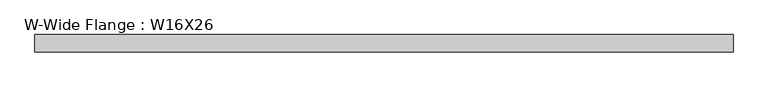
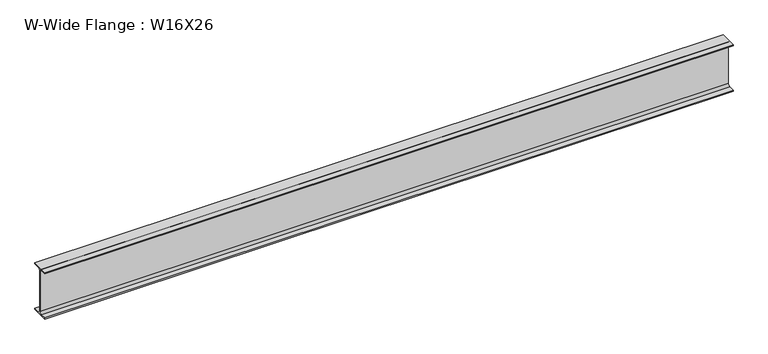
"""IFC4 building model written with IfcOpenShell, lengths in millimetres: beam geometry, W-Wide Flange : W16X26."""

from ifc_helpers import new_model, si_unit, point, frame, frame_2d, origin, place, context, project, spatial, polyline, circle_curve, trimmed, segment, composite_curve, outline, extrude, source, transform, mapped, element, save


def w_wide_flange_w16x26_811e96eb(model_context):
    return source(origin(), model_context, "Body", "SweptSolid", [
        extrude(outline(composite_curve([segment(polyline([(69.85, -190.627), (69.85, -199.39), (-69.85, -199.39), (-69.85, -190.627), (-21.3995, -190.627)]), True, "CONTINUOUS"), segment(trimmed(circle_curve(frame_2d((-21.3995, -172.4025)), 18.2245), [point((-21.3995, -190.627))], [point((-3.175, -172.4025))], True, "CARTESIAN"), True, "CONTINUOUS"), segment(polyline([(-3.175, -172.4025), (-3.175, 172.4025)]), True, "CONTINUOUS"), segment(trimmed(circle_curve(frame_2d((-21.3995, 172.4025)), 18.2245), [point((-3.175, 172.4025))], [point((-21.3995, 190.627))], True, "CARTESIAN"), True, "CONTINUOUS"), segment(polyline([(-21.3995, 190.627), (-69.85, 190.627), (-69.85, 199.39), (69.85, 199.39), (69.85, 190.627), (21.3995, 190.627)]), True, "CONTINUOUS"), segment(trimmed(circle_curve(frame_2d((21.3995, 172.4025)), 18.2245), [point((21.3995, 190.627))], [point((3.175, 172.4025))], True, "CARTESIAN"), True, "CONTINUOUS"), segment(polyline([(3.175, 172.4025), (3.175, -172.4025)]), True, "CONTINUOUS"), segment(trimmed(circle_curve(frame_2d((21.3995, -172.4025)), 18.2245), [point((3.175, -172.4025))], [point((21.3995, -190.627))], True, "CARTESIAN"), True, "CONTINUOUS"), segment(polyline([(21.3995, -190.627), (69.85, -190.627)]), True, "CONTINUOUS")], self_intersect=False)), frame((-2744.7378906, 0.0, 0.0), z_axis=(1.0, 0.0, 0.0), x_axis=(0.0, 1.0, 0.0)), (0.0, 0.0, 1.0), 5603.8253906),
    ])


if __name__ == "__main__":
    model = new_model("IFC4")
    model_context = context("Model", 3, world=origin())
    ifc_project = project(units=[si_unit("LENGTHUNIT", "METRE", prefix="MILLI")], contexts=[model_context])
    site = spatial("IfcSite", under=ifc_project)
    building = spatial("IfcBuilding", under=site)
    placement = place(None, origin())
    w_wide_flange_w16x26_shape = w_wide_flange_w16x26_811e96eb(model_context)
    element("IfcBeam", 1, ObjectType="W-Wide Flange : W16X26", at=placement, inside=building, context=model_context, shape_type="MappedRepresentation", body=[
        mapped(w_wide_flange_w16x26_shape, transform((0.0, 0.0, 0.0), x_axis=(1.0, 0.0, 0.0), y_axis=(0.0, 1.0, 0.0), z_axis=(0.0, 0.0, 1.0))),
    ])
    save(model, "model.ifc")

# Revit data of these elements
# Type "W-Wide Flange : W16X26"
#   Assembly Code = "B10"
#   W = 26
#   Length [instance default] = 1524 mm
#   bf = 139.7 mm
#   d = 398.78 mm
#   k = 26.988 mm
#   k2 = 18.225 mm
#   tf = 8.763 mm
#   tw = 6.35 mm
#   A = 0.00495483 m²
#   Structural Material [instance default] = Steel ASTM A992
# Element 1 (IfcBeam, "W-Wide Flange : W16X26")
#   Structural Material = Aluminum, Anodized Red
#   Materials on its faces: "Aluminum, Anodized Red"
# Materials
#   "Steel ASTM A992": class "Metal", colour RGB 128 0 0, transparency 0, Description = "Structural steel 50ksi", Cost = 0
#   "Aluminum, Anodized Red": class "Metal", colour RGB 120 120 120, transparency 0, Description = "Anodized aluminum, red", Cost = 0
